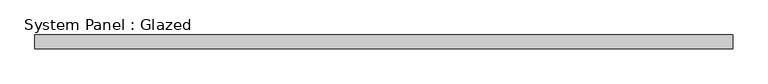
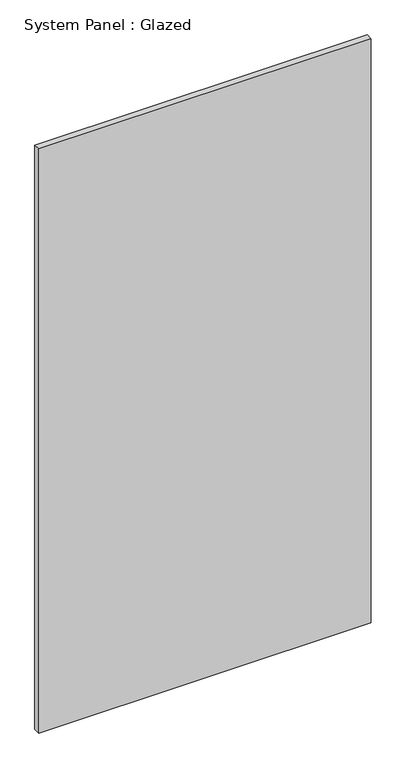
"""IFC4 building model written with IfcOpenShell, lengths in millimetres: plate geometry, System Panel : Glazed."""

from ifc_helpers import new_model, si_unit, origin, origin_with_axes, place, context, project, spatial, polyline, outline, extrude, source, transform, mapped, element, save


def system_panel_glazed_a88fc5f3(model_context):
    return source(origin(), model_context, "Body", "SweptSolid", [
        extrude(outline(polyline([(633.0541355, 24.5), (-633.0541355, 24.5), (-633.0541355, 49.5), (633.0541355, 49.5), (633.0541355, 24.5)])), origin_with_axes(), (0.0, 0.0, 1.0), 2350.0),
    ])


if __name__ == "__main__":
    model = new_model("IFC4")
    model_context = context("Model", 3, world=origin())
    ifc_project = project(units=[si_unit("LENGTHUNIT", "METRE", prefix="MILLI")], contexts=[model_context])
    site = spatial("IfcSite", under=ifc_project)
    building = spatial("IfcBuilding", under=site)
    placement = place(None, origin())
    system_panel_glazed_shape = system_panel_glazed_a88fc5f3(model_context)
    element("IfcPlate", 1, ObjectType="System Panel : Glazed", at=placement, inside=building, context=model_context, shape_type="MappedRepresentation", body=[
        mapped(system_panel_glazed_shape, transform((0.0, 0.0, 0.0), x_axis=(1.0, 0.0, 0.0), y_axis=(0.0, 1.0, 0.0), z_axis=(0.0, 0.0, 1.0))),
    ])
    save(model, "model.ifc")

# Revit data of these elements
# Type "System Panel : Glazed"
#   Construction Type Id = "GSP4R"
#   Analytic Construction = "1/8 in Pilkington single glazing"
#   Visual Light Transmittance = 0.9
#   Solar Heat Gain Coefficient = 0.86
#   Heat Transfer Coefficient (U) = 6.7069 W/(m²·K)
#   Define Thermal Properties by = 1
# Element 1 (IfcPlate, "System Panel : Glazed")
#   Materials on its faces: "Glass"
# Materials
#   "Glass": class "Glass", colour RGB 0 128 192, transparency 0.9, Description = "Soda Lime Glass", Cost = 0
